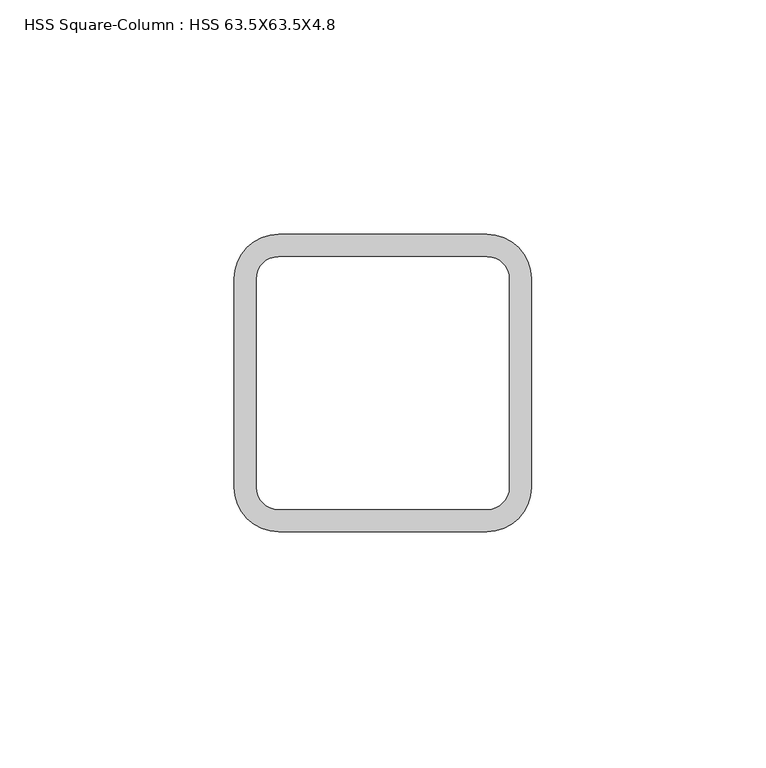
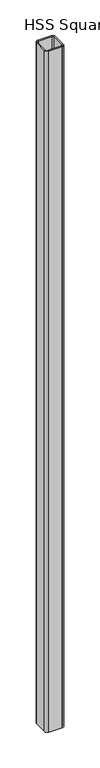
"""IFC4 building model written with IfcOpenShell, lengths in millimetres: column geometry, HSS Square-Column : HSS 63.5X63.5X4.8."""

from ifc_helpers import new_model, si_unit, point, frame, frame_2d, origin, place, context, project, spatial, polyline, circle_curve, trimmed, segment, composite_curve, outline, extrude, source, transform, mapped, element, save


def hss_square_column_hss_63_5x63_5x4_8_399af560(model_context):
    return source(origin(), model_context, "Body", "SweptSolid", [
        extrude(outline(composite_curve([segment(trimmed(circle_curve(frame_2d((22.225, 22.225)), 9.525), [point((22.225, 31.75))], [point((31.75, 22.225))], False, "CARTESIAN"), True, "CONTINUOUS"), segment(polyline([(31.75, 22.225), (31.75, -22.225)]), True, "CONTINUOUS"), segment(trimmed(circle_curve(frame_2d((22.225, -22.225)), 9.525), [point((31.75, -22.225))], [point((22.225, -31.75))], False, "CARTESIAN"), True, "CONTINUOUS"), segment(polyline([(22.225, -31.75), (-22.225, -31.75)]), True, "CONTINUOUS"), segment(trimmed(circle_curve(frame_2d((-22.225, -22.225)), 9.525), [point((-22.225, -31.75))], [point((-31.75, -22.225))], False, "CARTESIAN"), True, "CONTINUOUS"), segment(polyline([(-31.75, -22.225), (-31.75, 22.225)]), True, "CONTINUOUS"), segment(trimmed(circle_curve(frame_2d((-22.225, 22.225)), 9.525), [point((-31.75, 22.225))], [point((-22.225, 31.75))], False, "CARTESIAN"), True, "CONTINUOUS"), segment(polyline([(-22.225, 31.75), (22.225, 31.75)]), True, "CONTINUOUS")], self_intersect=False), holes=[composite_curve([segment(polyline([(22.225, 26.9875), (-22.225, 26.9875)]), True, "CONTINUOUS"), segment(trimmed(circle_curve(frame_2d((-22.225, 22.225)), 4.7625), [point((-22.225, 26.9875))], [point((-26.9875, 22.225))], True, "CARTESIAN"), True, "CONTINUOUS"), segment(polyline([(-26.9875, 22.225), (-26.9875, -22.225)]), True, "CONTINUOUS"), segment(trimmed(circle_curve(frame_2d((-22.225, -22.225)), 4.7625), [point((-26.9875, -22.225))], [point((-22.225, -26.9875))], True, "CARTESIAN"), True, "CONTINUOUS"), segment(polyline([(-22.225, -26.9875), (22.225, -26.9875)]), True, "CONTINUOUS"), segment(trimmed(circle_curve(frame_2d((22.225, -22.225)), 4.7625), [point((22.225, -26.9875))], [point((26.9875, -22.225))], True, "CARTESIAN"), True, "CONTINUOUS"), segment(polyline([(26.9875, -22.225), (26.9875, 22.225)]), True, "CONTINUOUS"), segment(trimmed(circle_curve(frame_2d((22.225, 22.225)), 4.7625), [point((26.9875, 22.225))], [point((22.225, 26.9875))], True, "CARTESIAN"), True, "CONTINUOUS")], self_intersect=False)]), frame((0.0, 0.0, 6240.0), z_axis=(0.0, 0.0, 1.0), x_axis=(1.0, 0.0, 0.0)), (0.0, 0.0, 1.0), 2400.0),
    ])


if __name__ == "__main__":
    model = new_model("IFC4")
    model_context = context("Model", 3, world=origin())
    ifc_project = project(units=[si_unit("LENGTHUNIT", "METRE", prefix="MILLI")], contexts=[model_context])
    site = spatial("IfcSite", under=ifc_project)
    building = spatial("IfcBuilding", under=site)
    placement = place(None, origin())
    hss_square_column_hss_63_5x63_5x4_8_shape = hss_square_column_hss_63_5x63_5x4_8_399af560(model_context)
    element("IfcColumn", 1, ObjectType="HSS Square-Column : HSS 63.5X63.5X4.8", at=placement, inside=building, context=model_context, shape_type="MappedRepresentation", body=[
        mapped(hss_square_column_hss_63_5x63_5x4_8_shape, transform((0.0, 0.0, 0.0), x_axis=(1.0, 0.0, 0.0), y_axis=(0.0, 1.0, 0.0), z_axis=(0.0, 0.0, 1.0))),
    ])
    save(model, "model.ifc")

# Revit data of these elements
# Type "HSS Square-Column : HSS 63.5X63.5X4.8"
#   Section Name Key = "HSS 2 1/2X2 1/2X3/16"
#   Assembly Code = "B10"
#   Width = 6.35 cm
#   Wall Nominal Thickness = 0.4763 cm
#   Wall Design Thickness = 0.442 cm
#   Torsional Moment of Inertia = 93.6521 cm⁴
#   Torsional Modulus = 30.4799 cm³
#   Section Area = 9.93546 cm²
#   Plastic Modulus weak axis = 21.6309 cm³
#   Plastic Modulus strong axis = 21.6309 cm³
#   Outer Fillet = 0.9525 cm
#   Nominal Weight = 8.31884 kgf/m
#   Moment of Inertia weak axis = 56.1912 cm⁴
#   Moment of Inertia strong axis = 56.1912 cm⁴
#   Inner Fillet = 0.4763 cm
#   Height = 6.35 cm
#   Elastic Modulus weak axis = 17.698 cm³
#   Elastic Modulus strong axis = 17.698 cm³
#   Centroid Vertical = 3.175 cm
#   Centroid Horizontal = 3.175 cm
#   Structural Material [instance default] = Steel ASTM A500, Grade B, Rectangular and Square
#   Principal Axes Angle = 0
# Element 1 (IfcColumn, "HSS Square-Column : HSS 63.5X63.5X4.8")
#   Structural Material = none
# Materials
#   "Steel ASTM A500, Grade B, Rectangular and Square": class "Metal", colour RGB 199 199 199, transparency 0, Description = "Carbon steel", Cost = 0
